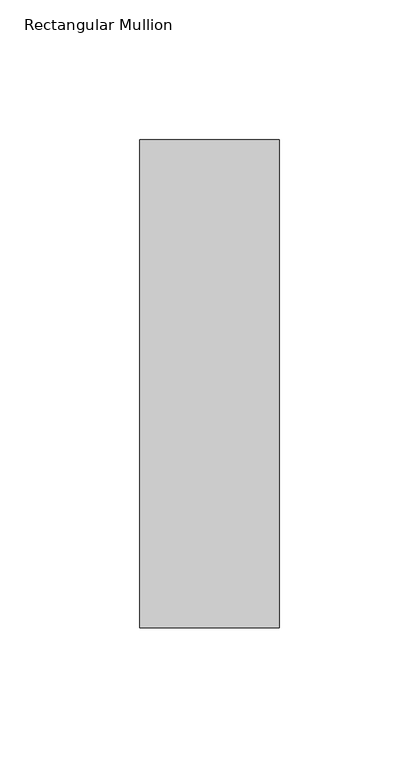
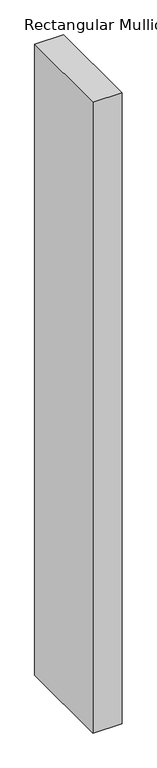
"""IFC4 building model written with IfcOpenShell, lengths in millimetres: member geometry, Rectangular Mullion : WWm-50x175-50mmOffset."""

import ifcopenshell
import ifcopenshell.guid

model = None  # the IFC model being written
_history = None  # IfcOwnerHistory: only IFC2X3 demands one
_inside = {}  # id of a spatial element -> (the spatial element, [elements in it])
_under = {}  # id of a project, library or spatial element -> (it, [spatial elements below it])
_declared = {}  # id of a project -> (the project, [libraries it declares])
_typed = {}  # id of a type object -> (the type object, [elements of that type])
_made_of = {}  # id of a material, layer set ... -> (it, [elements and type objects made of it])


def new_model(schema):
    """Start an empty IFC model of exactly this schema.

    Asked for "IFC4X3", IfcOpenShell would pick the latest addendum, in which some entities
    have other attributes; the version numbers below select the first issue.
    IFC2X3 requires an IfcOwnerHistory on every rooted entity: one is made here for all.
    """
    global model, _history
    if schema == "IFC4X3":
        model = ifcopenshell.file(schema_version=(4, 3, 0, 0))
    else:
        model = ifcopenshell.file(schema=schema)
    _inside.clear()
    _under.clear()
    _declared.clear()
    _typed.clear()
    _made_of.clear()
    _history = None
    if model.schema == "IFC2X3":
        org = make("IfcOrganization", Name="unknown")
        user = make(
            "IfcPersonAndOrganization",
            ThePerson=make("IfcPerson", FamilyName="unknown"),
            TheOrganization=org,
        )
        app = make(
            "IfcApplication",
            ApplicationDeveloper=org,
            Version="unknown",
            ApplicationFullName="unknown",
            ApplicationIdentifier="unknown",
        )
        _history = make(
            "IfcOwnerHistory",
            OwningUser=user,
            OwningApplication=app,
            ChangeAction="ADDED",
            CreationDate=0,
        )
    return model


def make(cls, **values):
    """One entity of the class cls with the attributes given. An attribute that is None is left unset."""
    return model.create_entity(
        cls, **{name: value for name, value in values.items() if value is not None}
    )


def rooted(cls, **values):
    """An entity with a GlobalId (a new one), such as an element, a storey or a relation."""
    return make(cls, GlobalId=ifcopenshell.guid.new(), OwnerHistory=_history, **values)


def si_unit(unit_type, name, prefix=None):
    """IfcSIUnit, for example si_unit("LENGTHUNIT", "METRE", prefix="MILLI")."""
    return make("IfcSIUnit", UnitType=unit_type, Prefix=prefix, Name=name)


def assignment(units):
    """IfcUnitAssignment: the units of a project."""
    return None if units is None else make("IfcUnitAssignment", Units=units)


def point(xyz):
    """IfcCartesianPoint."""
    return None if xyz is None else make("IfcCartesianPoint", Coordinates=xyz)


def direction(xyz):
    """IfcDirection."""
    return None if xyz is None else make("IfcDirection", DirectionRatios=xyz)


def frame(location, z_axis=None, x_axis=None):
    """IfcAxis2Placement3D, a coordinate frame: its origin and axes. An axis left out is left unset."""
    return make(
        "IfcAxis2Placement3D",
        Location=point(location),
        Axis=direction(z_axis),
        RefDirection=direction(x_axis),
    )


def origin():
    """The frame at (0, 0, 0) with its axes left unset."""
    return frame((0.0, 0.0, 0.0))


def place(relative_to, where):
    """IfcLocalPlacement: puts the frame where relative to a parent placement (None: the world)."""
    return make(
        "IfcLocalPlacement", PlacementRelTo=relative_to, RelativePlacement=where
    )


def context(
    kind, dimensions, precision=None, world=None, true_north=None, identifier=None
):
    """IfcGeometricRepresentationContext, for example the 3D "Model" context."""
    return make(
        "IfcGeometricRepresentationContext",
        ContextIdentifier=identifier,
        ContextType=kind,
        CoordinateSpaceDimension=dimensions,
        Precision=precision,
        WorldCoordinateSystem=world,
        TrueNorth=true_north,
    )


def project(units=None, contexts=None):
    """IfcProject with its units and contexts."""
    return rooted(
        "IfcProject",
        Name="project",
        RepresentationContexts=contexts,
        UnitsInContext=assignment(units),
    )


def spatial(cls, under=None, at=None, **own):
    """A site, building, storey or space (cls), placed at a placement, below another one or the project."""
    s = rooted(cls, ObjectPlacement=at, **own)
    if under is not None:
        _under.setdefault(under.id(), (under, []))[1].append(s)
    return s


def polyline(points):
    """IfcPolyline through the points."""
    return make("IfcPolyline", Points=[point(p) for p in points])


def outline(outer, holes=None, kind="AREA"):
    """IfcArbitraryClosedProfileDef: a profile drawn as a closed curve; with holes, ...WithVoids."""
    if holes is None:
        return make("IfcArbitraryClosedProfileDef", ProfileType=kind, OuterCurve=outer)
    return make(
        "IfcArbitraryProfileDefWithVoids",
        ProfileType=kind,
        OuterCurve=outer,
        InnerCurves=holes,
    )


def extrude(swept, where, along, depth):
    """IfcExtrudedAreaSolid: the profile swept, set in the frame where, extruded along a direction by depth."""
    return make(
        "IfcExtrudedAreaSolid",
        SweptArea=swept,
        Position=where,
        ExtrudedDirection=direction(along),
        Depth=depth,
    )


def shape(context_of_items, identifier, shape_type, items):
    """IfcShapeRepresentation: the items that make up one representation, for example the "Body"."""
    return make(
        "IfcShapeRepresentation",
        ContextOfItems=context_of_items,
        RepresentationIdentifier=identifier,
        RepresentationType=shape_type,
        Items=items,
    )


def source(mapping_origin, context_of_items, identifier, shape_type, items):
    """IfcRepresentationMap: a shape defined once, which mapped items show again and again."""
    return make(
        "IfcRepresentationMap",
        MappingOrigin=mapping_origin,
        MappedRepresentation=shape(context_of_items, identifier, shape_type, items),
    )


def transform(
    local_origin,
    x_axis=None,
    y_axis=None,
    z_axis=None,
    scale=None,
    scale2=None,
    scale3=None,
    uniform=True,
):
    """IfcCartesianTransformationOperator3D, or its non-uniform kind. x_axis, y_axis, z_axis: its Axis1, 2, 3."""
    if uniform:
        return make(
            "IfcCartesianTransformationOperator3D",
            Axis1=direction(x_axis),
            Axis2=direction(y_axis),
            LocalOrigin=point(local_origin),
            Scale=scale,
            Axis3=direction(z_axis),
        )
    return make(
        "IfcCartesianTransformationOperator3DnonUniform",
        Axis1=direction(x_axis),
        Axis2=direction(y_axis),
        LocalOrigin=point(local_origin),
        Scale=scale,
        Axis3=direction(z_axis),
        Scale2=scale2,
        Scale3=scale3,
    )


def mapped(mapping_source, mapping_target):
    """IfcMappedItem: shows the shape of a source again, moved by a transform."""
    return make(
        "IfcMappedItem", MappingSource=mapping_source, MappingTarget=mapping_target
    )


def made_of(thing, what):
    """Note that an element or type object is made of a material, layer set ...; save() writes the relation."""
    if what is not None:
        _made_of.setdefault(what.id(), (what, []))[1].append(thing)
    return thing


def element(
    cls,
    number,
    at=None,
    inside=None,
    cuts=None,
    type_object=None,
    material=None,
    context=None,
    identifier="Body",
    shape_type=None,
    held_by="IfcProductDefinitionShape",
    body=None,
    shapes=None,
    **own,
):
    """One element of the class cls, such as IfcWall. Its Tag is "e" and its number.

    at: its placement. inside: the storey or other place that contains it. cuts: it is an
    opening in that element (IfcRelVoidsElement). A single representation is given by context,
    identifier, shape_type and body (its items); several are given by shapes. held_by: the class
    of the entity that holds the representations. save() writes the other relations.
    """
    e = rooted(cls, Tag="e%d" % number, ObjectPlacement=at, **own)
    if body is not None:
        shapes = [shape(context, identifier, shape_type, body)]
    if shapes is not None:
        e.Representation = make(held_by, Representations=shapes)
    if inside is not None:
        _inside.setdefault(inside.id(), (inside, []))[1].append(e)
    if cuts is not None:
        rooted(
            "IfcRelVoidsElement", RelatingBuildingElement=cuts, RelatedOpeningElement=e
        )
    if type_object is not None:
        _typed.setdefault(type_object.id(), (type_object, []))[1].append(e)
    return made_of(e, material)


def aggregate(whole, parts):
    """IfcRelAggregates: a whole, such as a stair, and the parts it consists of."""
    return rooted("IfcRelAggregates", RelatingObject=whole, RelatedObjects=parts)


def save(model, path):
    """Write the relations noted so far, then the file.

    IfcRelAggregates (storeys below a building ...), IfcRelContainedInSpatialStructure (elements
    in a storey), IfcRelDefinesByType, IfcRelAssociatesMaterial and IfcRelDeclares: one each for
    every whole, place, type object, material and project.
    """
    for whole, parts in _under.values():
        aggregate(whole, parts)
    for where, things in _inside.values():
        rooted(
            "IfcRelContainedInSpatialStructure",
            RelatedElements=things,
            RelatingStructure=where,
        )
    for kind, things in _typed.values():
        rooted("IfcRelDefinesByType", RelatedObjects=things, RelatingType=kind)
    for what, things in _made_of.values():
        rooted("IfcRelAssociatesMaterial", RelatedObjects=things, RelatingMaterial=what)
    for by, libraries in _declared.values():
        rooted("IfcRelDeclares", RelatingContext=by, RelatedDefinitions=libraries)
    model.write(path)


def rectangular_mullion_1633b7e8(model_context):
    return source(origin(), model_context, "Body", "SweptSolid", [
        extrude(outline(polyline([(0.0, 87.5), (0.0, -87.5), (-50.0, -87.5), (-50.0, 87.5), (0.0, 87.5)])), frame((0.0, 0.0, -1155.0), z_axis=(0.0, 0.0, 1.0), x_axis=(1.0, 0.0, 0.0)), (0.0, 0.0, 1.0), 1155.0),
    ])


if __name__ == "__main__":
    model = new_model("IFC4")
    model_context = context("Model", 3, world=origin())
    ifc_project = project(units=[si_unit("LENGTHUNIT", "METRE", prefix="MILLI")], contexts=[model_context])
    site = spatial("IfcSite", under=ifc_project)
    building = spatial("IfcBuilding", under=site)
    placement = place(None, origin())
    rectangular_mullion_shape = rectangular_mullion_1633b7e8(model_context)
    element("IfcMember", 1, ObjectType="Rectangular Mullion : WWm-50x175-50mmOffset", at=placement, inside=building, context=model_context, shape_type="MappedRepresentation", body=[
        mapped(rectangular_mullion_shape, transform((0.0, 0.0, 0.0), x_axis=(1.0, 0.0, 0.0), y_axis=(0.0, 1.0, 0.0), z_axis=(0.0, 0.0, 1.0))),
    ])
    save(model, "model.ifc")

# Revit data of these elements
# Type "Rectangular Mullion : WWm-50x175-50mmOffset"
#   built-in parameter 1007304 = 0.574147 (stored number, unit not read)
#   built-in parameter 1007301 = 0.082021 (stored number, unit not read)
#   built-in parameter 1007300 = 0.082021 (stored number, unit not read)
# Element 1 (IfcMember, "Rectangular Mullion : WWm-50x175-50mmOffset")
#   Materials on its faces: "WW-EC-RGB-Mullion"
# Materials
#   "WW-EC-RGB-Mullion": class "Generic", colour RGB 255 255 255, transparency 0, Comments = "If region requests black mullions, switch asset color to RGB 25-25-25", Description = "Generic Color", Cost = 0
